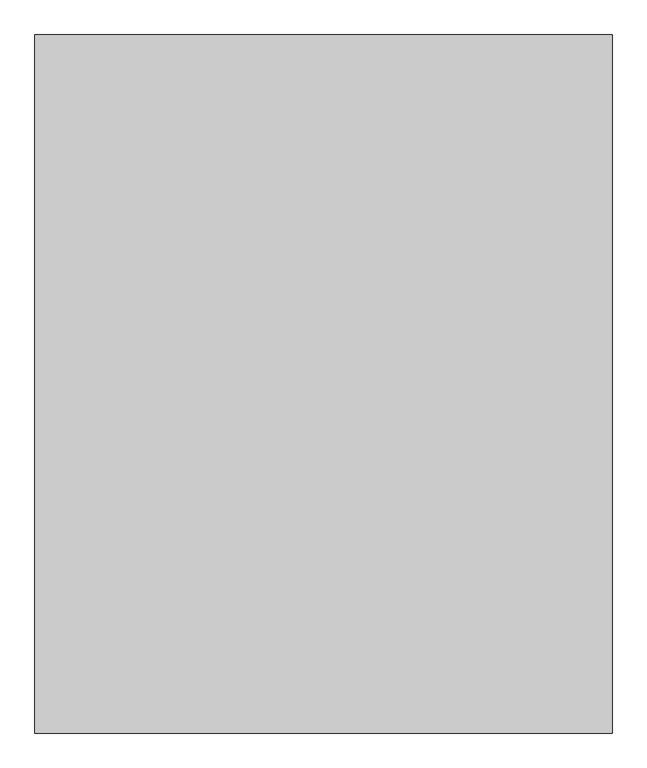
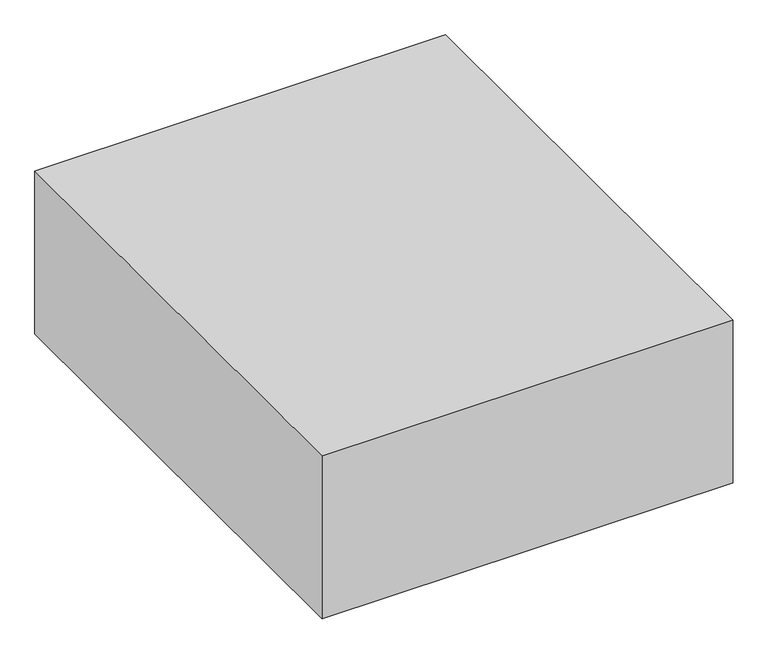
"""IFC4 building model written with IfcOpenShell, lengths in millimetres: proxy geometry, Space Planning Box_hec : Space Planning Box_hec."""

from ifc_helpers import new_model, si_unit, origin, origin_with_axes, place, context, project, spatial, polyline, outline, extrude, source, transform, mapped, element, save


def generic_models_246d78d5(model_context):
    return source(origin(), model_context, "Body", "SweptSolid", [
        extrude(outline(polyline([(6200.0, 7500.0), (6200.0, -7500.0), (-6200.0, -7500.0), (-6200.0, 7500.0), (6200.0, 7500.0)])), origin_with_axes(), (0.0, 0.0, 1.0), 5200.0),
    ])


if __name__ == "__main__":
    model = new_model("IFC4")
    model_context = context("Model", 3, world=origin())
    ifc_project = project(units=[si_unit("LENGTHUNIT", "METRE", prefix="MILLI")], contexts=[model_context])
    site = spatial("IfcSite", under=ifc_project)
    building = spatial("IfcBuilding", under=site)
    placement = place(None, origin())
    generic_models_shape = generic_models_246d78d5(model_context)
    element("IfcBuildingElementProxy", 1, Name="Space Planning Box_hec : Space Planning Box_hec", ObjectType="Space Planning Box_hec : Space Planning Box_hec", at=placement, inside=building, context=model_context, shape_type="MappedRepresentation", body=[
        mapped(generic_models_shape, transform((0.0, 0.0, 0.0), x_axis=(1.0, 0.0, 0.0), y_axis=(0.0, 1.0, 0.0), z_axis=(0.0, 0.0, 1.0))),
    ])
    save(model, "model.ifc")

# Revit data of these elements
# Type "Space Planning Box_hec : Space Planning Box_hec"
#   Type Comments = "..."
#   Room Name [instance default] = "?"
#   Interior Finish [instance default] = ""
#   Exterior Finish [instance default] = ""
#   Department [instance default] = ""
#   Assembly Code = "..."
#   ceiling height [instance default] = 0
#   Width [instance default] = 1524 mm
#   Program Area [instance default] = 0.00 m²
#   Length [instance default] = 1524 mm
#   Height [instance default] = 1524 mm
#   Area [instance default] = 2.32258 m²
#   Fill Color [instance default] = Cyan
#   Default Elevation = 0
# Element 1 (IfcBuildingElementProxy, "Space Planning Box_hec : Space Planning Box_hec")
#   Room Name = "Central Control Room"
#   Interior Finish = "IW1..N/A,,WB2..N/A,,FL7..N/A,,CL4..N/A"
#   Exterior Finish = "N/A..N/A,,EW1..N/A"
#   Department = "CI"
#   ceiling height = 3400
#   Width = 12400 mm
#   Program Area = 186.00 m²
#   Length = 15000 mm
#   Height = 5200 mm
#   Area = 186.00 m²
#   Fill Color = Yellow
#   Materials on its faces: "Yellow"
# Materials
#   "Cyan": class "Generic", colour RGB 0 255 255, transparency 0.2, Cost = 0
#   "Yellow": class "Generic", colour RGB 255 255 0, transparency 0.2, Cost = 0
